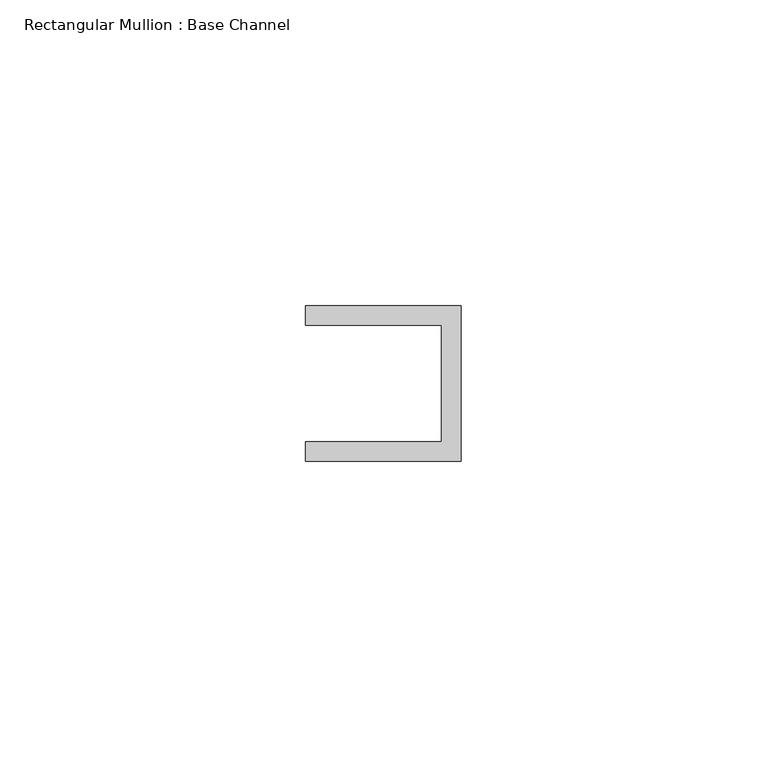
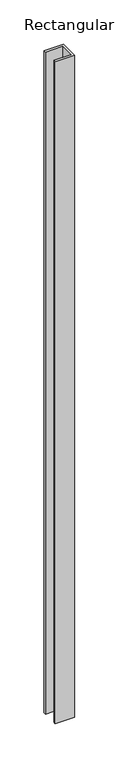
"""IFC4 building model written with IfcOpenShell, lengths in millimetres: member geometry, Rectangular Mullion : Base Channel."""

from ifc_helpers import new_model, si_unit, frame, origin, place, context, project, spatial, polyline, outline, extrude, source, transform, mapped, element, save


def rectangular_mullion_base_channel_0014d07f(model_context):
    return source(origin(), model_context, "Body", "SweptSolid", [
        extrude(outline(polyline([(0.0, 12.7), (0.0, -12.7), (-25.4, -12.7), (-25.4, -9.525), (-3.175, -9.525), (-3.175, 9.525), (-25.4, 9.525), (-25.4, 12.7), (0.0, 12.7)])), frame((0.0, 0.0, -914.4), z_axis=(0.0, 0.0, 1.0), x_axis=(1.0, 0.0, 0.0)), (0.0, 0.0, 1.0), 914.4),
    ])


if __name__ == "__main__":
    model = new_model("IFC4")
    model_context = context("Model", 3, world=origin())
    ifc_project = project(units=[si_unit("LENGTHUNIT", "METRE", prefix="MILLI")], contexts=[model_context])
    site = spatial("IfcSite", under=ifc_project)
    building = spatial("IfcBuilding", under=site)
    placement = place(None, origin())
    rectangular_mullion_base_channel_shape = rectangular_mullion_base_channel_0014d07f(model_context)
    element("IfcMember", 1, ObjectType="Rectangular Mullion : Base Channel", at=placement, inside=building, context=model_context, shape_type="MappedRepresentation", body=[
        mapped(rectangular_mullion_base_channel_shape, transform((0.0, 0.0, 0.0), x_axis=(1.0, 0.0, 0.0), y_axis=(0.0, 1.0, 0.0), z_axis=(0.0, 0.0, 1.0))),
    ])
    save(model, "model.ifc")

# Revit data of these elements
# Project information
#   Project Issue Date = "11/01/2019"
#   Project Status = "Project Status"
#   Client Name = "Owner"
#   Project Address = "725 E JOHNSON ST. -  MADISON, WI"
#   Project Name = "PALISADE PROPERTY"
#   Project Number = "Project Number"
# Type "Rectangular Mullion : Base Channel"
#   built-in parameter 1007322 = 0.0833333 (stored number, unit not read)
#   built-in parameter 1007321 = 0.0416667 (stored number, unit not read)
#   built-in parameter 1007320 = -0.03125 (stored number, unit not read)
# Element 1 (IfcMember, "Rectangular Mullion : Base Channel")
#   Materials on its faces: "ALUM"
# Materials
#   "ALUM": class "Generic", colour RGB 157 157 157, transparency 0, Cost = 0
